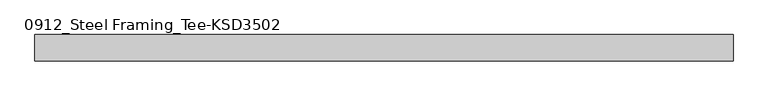
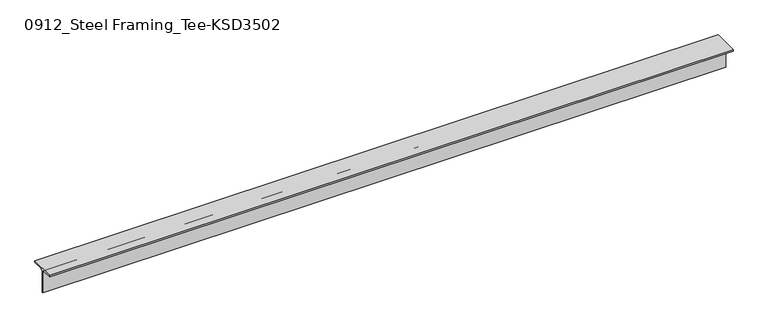
"""IFC4 building model written with IfcOpenShell, lengths in millimetres: member geometry, 0912_Steel Framing_Tee-KSD3502 : H_SB_ASB_CT-150x150x6.5x9."""

from ifc_helpers import new_model, si_unit, point, frame, frame_2d, origin, place, context, project, spatial, polyline, circle_curve, trimmed, segment, composite_curve, outline, extrude, source, transform, mapped, element, save


def member_0912_steel_framing_tee_ksd3502_ae2583ae(model_context):
    return source(origin(), model_context, "Body", "SweptSolid", [
        extrude(outline(composite_curve([segment(polyline([(-75.0, 75.0), (75.0, 75.0), (75.0, 66.0), (16.25, 66.0)]), True, "CONTINUOUS"), segment(trimmed(circle_curve(frame_2d((16.25, 53.0)), 13.0), [point((16.25, 66.0))], [point((3.25, 53.0))], True, "CARTESIAN"), True, "CONTINUOUS"), segment(polyline([(3.25, 53.0), (3.25, -75.0), (-3.25, -75.0), (-3.25, 53.0)]), True, "CONTINUOUS"), segment(trimmed(circle_curve(frame_2d((-16.25, 53.0)), 13.0), [point((-3.25, 53.0))], [point((-16.25, 66.0))], True, "CARTESIAN"), True, "CONTINUOUS"), segment(polyline([(-16.25, 66.0), (-75.0, 66.0), (-75.0, 75.0)]), True, "CONTINUOUS")], self_intersect=False)), frame((-2003.05, 0.0, 0.0), z_axis=(1.0, 0.0, 0.0), x_axis=(0.0, 1.0, 0.0)), (0.0, 0.0, 1.0), 3968.5),
    ])


if __name__ == "__main__":
    model = new_model("IFC4")
    model_context = context("Model", 3, world=origin())
    ifc_project = project(units=[si_unit("LENGTHUNIT", "METRE", prefix="MILLI")], contexts=[model_context])
    site = spatial("IfcSite", under=ifc_project)
    building = spatial("IfcBuilding", under=site)
    placement = place(None, origin())
    member_0912_steel_framing_tee_ksd3502_shape = member_0912_steel_framing_tee_ksd3502_ae2583ae(model_context)
    element("IfcMember", 1, ObjectType="0912_Steel Framing_Tee-KSD3502 : H_SB_ASB_CT-150x150x6.5x9", at=placement, inside=building, context=model_context, shape_type="MappedRepresentation", body=[
        mapped(member_0912_steel_framing_tee_ksd3502_shape, transform((0.0, 0.0, 0.0), x_axis=(1.0, 0.0, 0.0), y_axis=(0.0, 1.0, 0.0), z_axis=(0.0, 0.0, 1.0))),
    ])
    save(model, "model.ifc")

# Revit data of these elements
# Type "0912_Steel Framing_Tee-KSD3502 : H_SB_ASB_CT-150x150x6.5x9"
#   H_WM Code_1 = "S01AA003-00001 | Main Steel Structure Fabrication Work | Shelter/Building | Light Steel - Standard (30KG/M>Weight) | Material: (   )"
#   H_WM Code_2 = "S03AA029-00001 | Main Steel Structure Erection Work | Shelter/Building | Light Steel (30KG/M>Weight) | Material: (   )"
#   H_WM Code_3 = "S01AA010-00001 | Main Steel Structure Fabrication Work | Shelter/Building | Steel Painting/Coating | for Non-Fireproofed Steel Surface, Surface Preparation, Primer, Second & Final Coat | Material: (   )"
#   H_Q'ty Cal Type Tag = "SB-Q2"
#   Width = 15.0 cm
#   Web Thickness = 0.65 cm
#   Web Fillet = 1.3 cm
#   Section Area = 23.39 cm²
#   Perimeter = 0.60 m²/m
#   Nominal Weight = 18.40 kgf/m
#   Height = 15.0 cm
#   Flange Thickness = 0.9 cm
#   Centroid Vertical = 7.5 cm
#   Centroid Horizontal = 7.5 cm
#   Length [instance default] = 1.5000 m
#   Structural Material [instance default] = Steel, 45-345
#   Warping Constant = (empty or 0)
#   Torsional Moment of Inertia = 0
#   Section Name Key = ""
#   Plastic Modulus weak axis = 0
#   Plastic Modulus strong axis = 0
#   Moment of Inertia weak axis = 0
#   Moment of Inertia strong axis = 0
#   Elastic Modulus weak axis = 0
#   Elastic Modulus strong axis = 0
#   Bolt Spacing = 0
#   Assembly Code = ""
# Element 1 (IfcMember, "0912_Steel Framing_Tee-KSD3502 : H_SB_ASB_CT-150x150x6.5x9")
#   Structural Material = none
# Materials
#   "Steel, 45-345": class "Metal", colour RGB 189 187 185, transparency 0, Description = "Steel 345 MPa", Cost = 0
